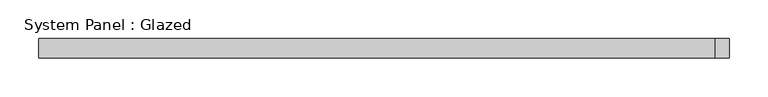
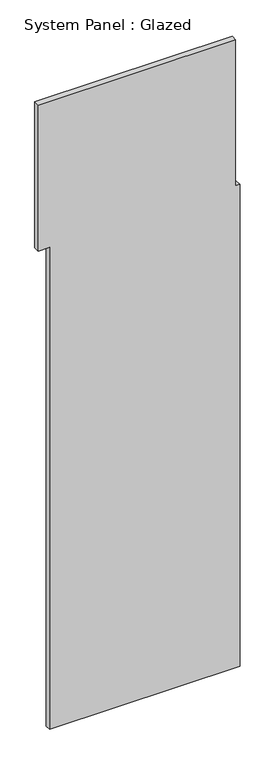
"""IFC4 building model written with IfcOpenShell, lengths in millimetres: plate geometry, System Panel : Glazed."""

from ifc_helpers import new_model, si_unit, frame, origin, place, context, project, spatial, polyline, outline, extrude, source, transform, mapped, element, save


def system_panel_glazed_ca088a96(model_context):
    return source(origin(), model_context, "Body", "SweptSolid", [
        extrude(outline(polyline([(0.0, -397.289433), (0.0, 448.089433), (2260.6, 448.089433), (2260.6, 429.039433), (2946.4, 429.039433), (2946.4, -448.089433), (2260.6, -448.089433), (2260.6, -397.289433), (0.0, -397.289433)])), frame((0.0, -12.7, 0.0), z_axis=(0.0, 1.0, 0.0), x_axis=(0.0, 0.0, 1.0)), (0.0, 0.0, 1.0), 25.4),
    ])


if __name__ == "__main__":
    model = new_model("IFC4")
    model_context = context("Model", 3, world=origin())
    ifc_project = project(units=[si_unit("LENGTHUNIT", "METRE", prefix="MILLI")], contexts=[model_context])
    site = spatial("IfcSite", under=ifc_project)
    building = spatial("IfcBuilding", under=site)
    placement = place(None, origin())
    system_panel_glazed_shape = system_panel_glazed_ca088a96(model_context)
    element("IfcPlate", 1, ObjectType="System Panel : Glazed", at=placement, inside=building, context=model_context, shape_type="MappedRepresentation", body=[
        mapped(system_panel_glazed_shape, transform((0.0, 0.0, 0.0), x_axis=(1.0, 0.0, 0.0), y_axis=(0.0, 1.0, 0.0), z_axis=(0.0, 0.0, 1.0))),
    ])
    save(model, "model.ifc")

# Revit data of these elements
# Element 1 (IfcPlate, "System Panel : Glazed")
#   Materials on its faces: "BUTT GLAZED STOREFRONT WITH VERTICAL MULLION"
# Materials
#   "BUTT GLAZED STOREFRONT WITH VERTICAL MULLION": class "Glass", colour RGB 236 240 239, transparency 0.39, Description = "Soda Lime Glass", Cost = 0
